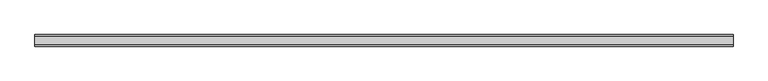
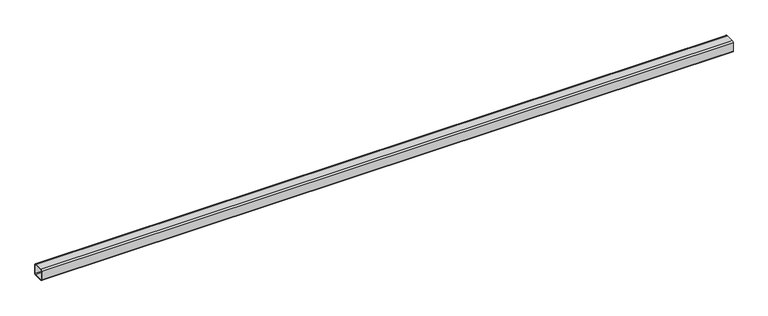
"""IFC4 building model written with IfcOpenShell, lengths in millimetres: beam geometry, Гнутый прямоугольный профиль (Трубы 30245-94) Балки : гнутый прямоуг. проф. 100x6."""

from ifc_helpers import new_model, si_unit, point, frame, frame_2d, origin, place, context, project, spatial, polyline, circle_curve, trimmed, segment, composite_curve, outline, extrude, source, transform, mapped, element, save


def beam_ec44c535(model_context):
    return source(origin(), model_context, "Body", "SweptSolid", [
        extrude(outline(composite_curve([segment(polyline([(-38.0, 50.0), (38.0, 50.0)]), True, "CONTINUOUS"), segment(trimmed(circle_curve(frame_2d((38.0, 38.0)), 12.0), [point((38.0, 50.0))], [point((50.0, 38.0))], False, "CARTESIAN"), True, "CONTINUOUS"), segment(polyline([(50.0, 38.0), (50.0, -38.0)]), True, "CONTINUOUS"), segment(trimmed(circle_curve(frame_2d((38.0, -38.0)), 12.0), [point((50.0, -38.0))], [point((38.0, -50.0))], False, "CARTESIAN"), True, "CONTINUOUS"), segment(polyline([(38.0, -50.0), (-38.0, -50.0)]), True, "CONTINUOUS"), segment(trimmed(circle_curve(frame_2d((-38.0, -38.0)), 12.0), [point((-38.0, -50.0))], [point((-50.0, -38.0))], False, "CARTESIAN"), True, "CONTINUOUS"), segment(polyline([(-50.0, -38.0), (-50.0, 38.0)]), True, "CONTINUOUS"), segment(trimmed(circle_curve(frame_2d((-38.0, 38.0)), 12.0), [point((-50.0, 38.0))], [point((-38.0, 50.0))], False, "CARTESIAN"), True, "CONTINUOUS")], self_intersect=False), holes=[composite_curve([segment(trimmed(circle_curve(frame_2d((-38.0, 38.0)), 6.0), [point((-38.0, 44.0))], [point((-44.0, 38.0))], True, "CARTESIAN"), True, "CONTINUOUS"), segment(polyline([(-44.0, 38.0), (-44.0, -38.0)]), True, "CONTINUOUS"), segment(trimmed(circle_curve(frame_2d((-38.0, -38.0)), 6.0), [point((-44.0, -38.0))], [point((-38.0, -44.0))], True, "CARTESIAN"), True, "CONTINUOUS"), segment(polyline([(-38.0, -44.0), (38.0, -44.0)]), True, "CONTINUOUS"), segment(trimmed(circle_curve(frame_2d((38.0, -38.0)), 6.0), [point((38.0, -44.0))], [point((44.0, -38.0))], True, "CARTESIAN"), True, "CONTINUOUS"), segment(polyline([(44.0, -38.0), (44.0, 38.0)]), True, "CONTINUOUS"), segment(trimmed(circle_curve(frame_2d((38.0, 38.0)), 6.0), [point((44.0, 38.0))], [point((38.0, 44.0))], True, "CARTESIAN"), True, "CONTINUOUS"), segment(polyline([(38.0, 44.0), (-38.0, 44.0)]), True, "CONTINUOUS")], self_intersect=False)]), frame((-3000.0, 0.0, 0.0), z_axis=(1.0, 0.0, 0.0), x_axis=(0.0, 1.0, 0.0)), (0.0, 0.0, 1.0), 6000.0),
    ])


if __name__ == "__main__":
    model = new_model("IFC4")
    model_context = context("Model", 3, world=origin())
    ifc_project = project(units=[si_unit("LENGTHUNIT", "METRE", prefix="MILLI")], contexts=[model_context])
    site = spatial("IfcSite", under=ifc_project)
    building = spatial("IfcBuilding", under=site)
    placement = place(None, origin())
    beam_shape = beam_ec44c535(model_context)
    element("IfcBeam", 1, ObjectType="Гнутый прямоугольный профиль (Трубы 30245-94) Балки : гнутый прямоуг. проф. 100x6", at=placement, inside=building, context=model_context, shape_type="MappedRepresentation", body=[
        mapped(beam_shape, transform((0.0, 0.0, 0.0), x_axis=(1.0, 0.0, 0.0), y_axis=(0.0, 1.0, 0.0), z_axis=(0.0, 0.0, 1.0))),
    ])
    save(model, "model.ifc")

# Revit data of these elements
# Type "Гнутый прямоугольный профиль (Трубы 30245-94) Балки : гнутый прямоуг. проф. 100x6"
#   ri = 12 mm
#   ra = 6 mm
#   W = 0.173578
#   Vz = 50 mm
#   Vy = 50 mm
#   Vpz = 50 mm
#   Vpy = 50 mm
#   Length [instance default] = 1500 mm
#   bf = 100 mm
#   d = 100 mm
#   tf = 6 mm
#   tw = 6 mm
#   A = 0.00226 m²
#   Structural Material [instance default] = Металл - Сталь - 345 МПa
#   Assembly Code = ""
# Element 1 (IfcBeam, "Гнутый прямоугольный профиль (Трубы 30245-94) Балки : гнутый прямоуг. проф. 100x6")
#   Structural Material = C235
#   Materials on its faces: "C235"
# Materials
#   "Металл - Сталь - 345 МПa": class "Металл", colour RGB 247 247 247, transparency 0
#   "C235": class "Не назначено", colour RGB 0 0 0, transparency 0
